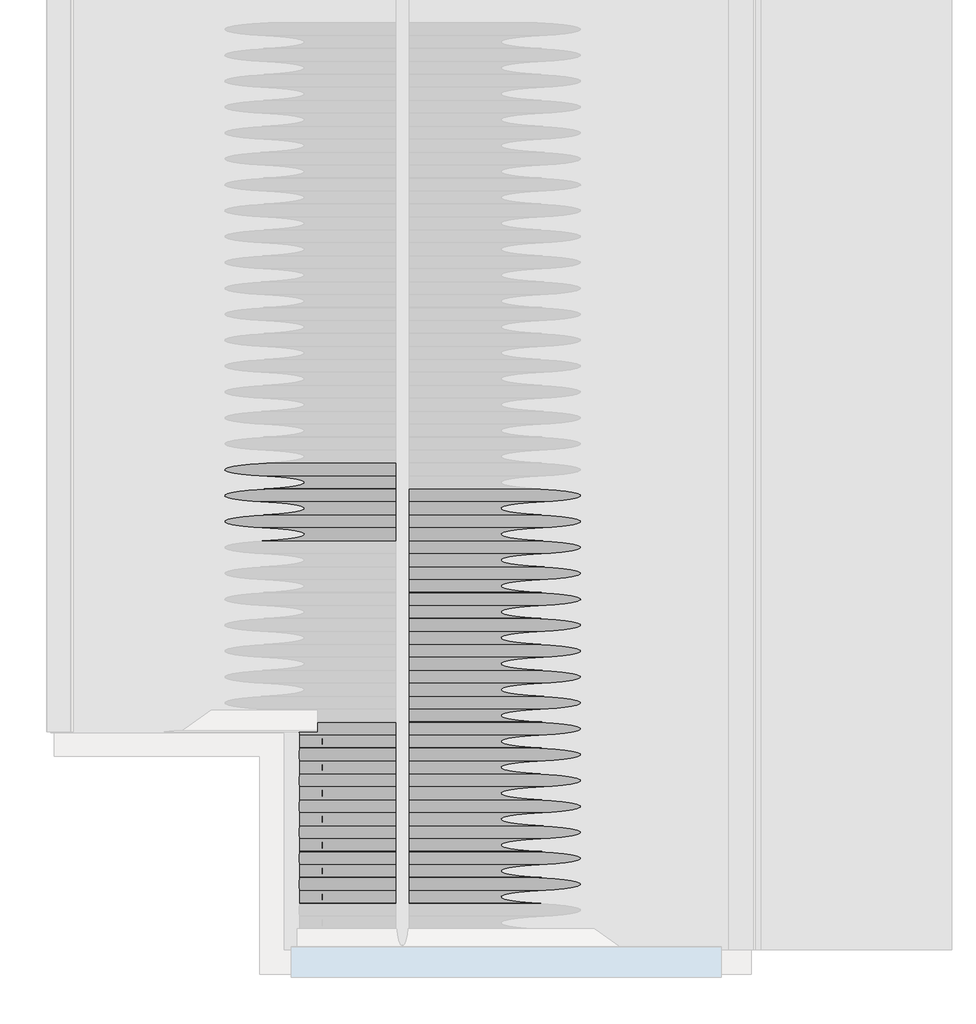
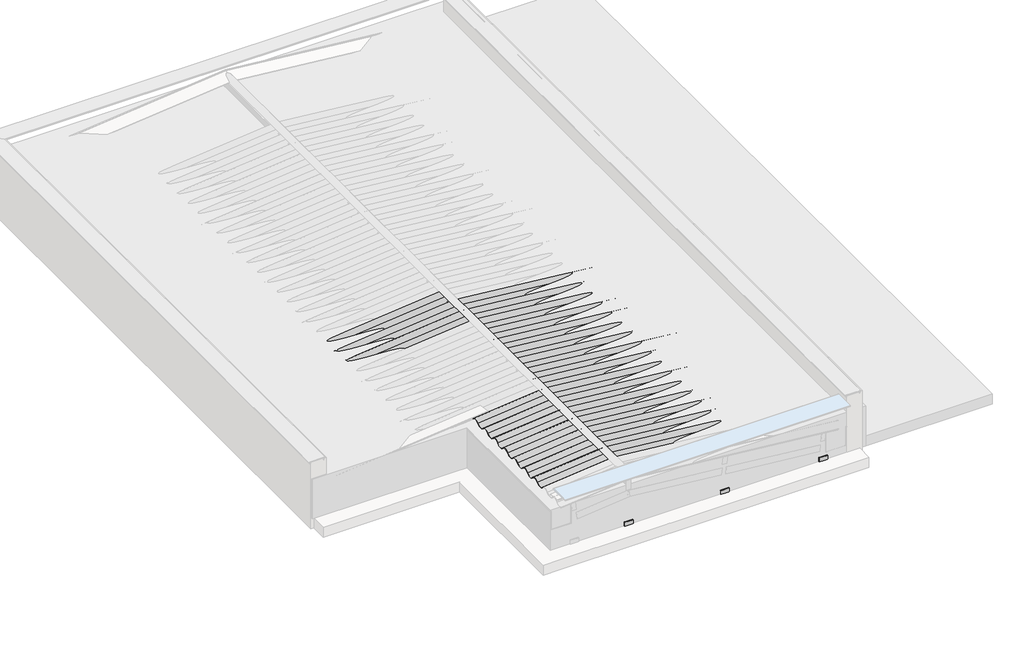
# One storey, part 2 of 4: 34 beams, 4 columns.
"""IFC4 building model written with IfcOpenShell, lengths in millimetres."""

import ifcopenshell
import ifcopenshell.guid

model = None  # the IFC model being written
_history = None  # IfcOwnerHistory: only IFC2X3 demands one
_inside = {}  # id of a spatial element -> (the spatial element, [elements in it])
_under = {}  # id of a project, library or spatial element -> (it, [spatial elements below it])
_declared = {}  # id of a project -> (the project, [libraries it declares])
_typed = {}  # id of a type object -> (the type object, [elements of that type])
_made_of = {}  # id of a material, layer set ... -> (it, [elements and type objects made of it])


def new_model(schema):
    """Start an empty IFC model of exactly this schema.

    Asked for "IFC4X3", IfcOpenShell would pick the latest addendum, in which some entities
    have other attributes; the version numbers below select the first issue.
    IFC2X3 requires an IfcOwnerHistory on every rooted entity: one is made here for all.
    """
    global model, _history
    if schema == "IFC4X3":
        model = ifcopenshell.file(schema_version=(4, 3, 0, 0))
    else:
        model = ifcopenshell.file(schema=schema)
    _inside.clear()
    _under.clear()
    _declared.clear()
    _typed.clear()
    _made_of.clear()
    _history = None
    if model.schema == "IFC2X3":
        org = make("IfcOrganization", Name="unknown")
        user = make(
            "IfcPersonAndOrganization",
            ThePerson=make("IfcPerson", FamilyName="unknown"),
            TheOrganization=org,
        )
        app = make(
            "IfcApplication",
            ApplicationDeveloper=org,
            Version="unknown",
            ApplicationFullName="unknown",
            ApplicationIdentifier="unknown",
        )
        _history = make(
            "IfcOwnerHistory",
            OwningUser=user,
            OwningApplication=app,
            ChangeAction="ADDED",
            CreationDate=0,
        )
    return model


def make(cls, **values):
    """One entity of the class cls with the attributes given. An attribute that is None is left unset."""
    return model.create_entity(
        cls, **{name: value for name, value in values.items() if value is not None}
    )


def rooted(cls, **values):
    """An entity with a GlobalId (a new one), such as an element, a storey or a relation."""
    return make(cls, GlobalId=ifcopenshell.guid.new(), OwnerHistory=_history, **values)


def si_unit(unit_type, name, prefix=None):
    """IfcSIUnit, for example si_unit("LENGTHUNIT", "METRE", prefix="MILLI")."""
    return make("IfcSIUnit", UnitType=unit_type, Prefix=prefix, Name=name)


def assignment(units):
    """IfcUnitAssignment: the units of a project."""
    return None if units is None else make("IfcUnitAssignment", Units=units)


def point(xyz):
    """IfcCartesianPoint."""
    return None if xyz is None else make("IfcCartesianPoint", Coordinates=xyz)


def direction(xyz):
    """IfcDirection."""
    return None if xyz is None else make("IfcDirection", DirectionRatios=xyz)


def frame(location, z_axis=None, x_axis=None):
    """IfcAxis2Placement3D, a coordinate frame: its origin and axes. An axis left out is left unset."""
    return make(
        "IfcAxis2Placement3D",
        Location=point(location),
        Axis=direction(z_axis),
        RefDirection=direction(x_axis),
    )


def frame_2d(location, x_axis=None):
    """IfcAxis2Placement2D, a coordinate frame in the plane: its origin and x axis."""
    return make(
        "IfcAxis2Placement2D", Location=point(location), RefDirection=direction(x_axis)
    )


def origin():
    """The frame at (0, 0, 0) with its axes left unset."""
    return frame((0.0, 0.0, 0.0))


def place(relative_to, where):
    """IfcLocalPlacement: puts the frame where relative to a parent placement (None: the world)."""
    return make(
        "IfcLocalPlacement", PlacementRelTo=relative_to, RelativePlacement=where
    )


def context(
    kind, dimensions, precision=None, world=None, true_north=None, identifier=None
):
    """IfcGeometricRepresentationContext, for example the 3D "Model" context."""
    return make(
        "IfcGeometricRepresentationContext",
        ContextIdentifier=identifier,
        ContextType=kind,
        CoordinateSpaceDimension=dimensions,
        Precision=precision,
        WorldCoordinateSystem=world,
        TrueNorth=true_north,
    )


def project(units=None, contexts=None):
    """IfcProject with its units and contexts."""
    return rooted(
        "IfcProject",
        Name="project",
        RepresentationContexts=contexts,
        UnitsInContext=assignment(units),
    )


def spatial(cls, under=None, at=None, **own):
    """A site, building, storey or space (cls), placed at a placement, below another one or the project."""
    s = rooted(cls, ObjectPlacement=at, **own)
    if under is not None:
        _under.setdefault(under.id(), (under, []))[1].append(s)
    return s


def polyline(points):
    """IfcPolyline through the points."""
    return make("IfcPolyline", Points=[point(p) for p in points])


def circle_curve(where, radius):
    """IfcCircle in the frame where."""
    return make("IfcCircle", Position=where, Radius=radius)


def trimmed(basis, trim1, trim2, sense, master):
    """IfcTrimmedCurve: the piece of a basis curve between two trims."""
    return make(
        "IfcTrimmedCurve",
        BasisCurve=basis,
        Trim1=trim1,
        Trim2=trim2,
        SenseAgreement=sense,
        MasterRepresentation=master,
    )


def segment(curve, same_sense, transition):
    """IfcCompositeCurveSegment."""
    return make(
        "IfcCompositeCurveSegment",
        Transition=transition,
        SameSense=same_sense,
        ParentCurve=curve,
    )


def composite_curve(segments, self_intersect=None):
    """IfcCompositeCurve: segments joined end to end."""
    return make("IfcCompositeCurve", Segments=segments, SelfIntersect=self_intersect)


def outline(outer, holes=None, kind="AREA"):
    """IfcArbitraryClosedProfileDef: a profile drawn as a closed curve; with holes, ...WithVoids."""
    if holes is None:
        return make("IfcArbitraryClosedProfileDef", ProfileType=kind, OuterCurve=outer)
    return make(
        "IfcArbitraryProfileDefWithVoids",
        ProfileType=kind,
        OuterCurve=outer,
        InnerCurves=holes,
    )


def extrude(swept, where, along, depth):
    """IfcExtrudedAreaSolid: the profile swept, set in the frame where, extruded along a direction by depth."""
    return make(
        "IfcExtrudedAreaSolid",
        SweptArea=swept,
        Position=where,
        ExtrudedDirection=direction(along),
        Depth=depth,
    )


def shape(context_of_items, identifier, shape_type, items):
    """IfcShapeRepresentation: the items that make up one representation, for example the "Body"."""
    return make(
        "IfcShapeRepresentation",
        ContextOfItems=context_of_items,
        RepresentationIdentifier=identifier,
        RepresentationType=shape_type,
        Items=items,
    )


def source(mapping_origin, context_of_items, identifier, shape_type, items):
    """IfcRepresentationMap: a shape defined once, which mapped items show again and again."""
    return make(
        "IfcRepresentationMap",
        MappingOrigin=mapping_origin,
        MappedRepresentation=shape(context_of_items, identifier, shape_type, items),
    )


def transform(
    local_origin,
    x_axis=None,
    y_axis=None,
    z_axis=None,
    scale=None,
    scale2=None,
    scale3=None,
    uniform=True,
):
    """IfcCartesianTransformationOperator3D, or its non-uniform kind. x_axis, y_axis, z_axis: its Axis1, 2, 3."""
    if uniform:
        return make(
            "IfcCartesianTransformationOperator3D",
            Axis1=direction(x_axis),
            Axis2=direction(y_axis),
            LocalOrigin=point(local_origin),
            Scale=scale,
            Axis3=direction(z_axis),
        )
    return make(
        "IfcCartesianTransformationOperator3DnonUniform",
        Axis1=direction(x_axis),
        Axis2=direction(y_axis),
        LocalOrigin=point(local_origin),
        Scale=scale,
        Axis3=direction(z_axis),
        Scale2=scale2,
        Scale3=scale3,
    )


def mapped(mapping_source, mapping_target):
    """IfcMappedItem: shows the shape of a source again, moved by a transform."""
    return make(
        "IfcMappedItem", MappingSource=mapping_source, MappingTarget=mapping_target
    )


def made_of(thing, what):
    """Note that an element or type object is made of a material, layer set ...; save() writes the relation."""
    if what is not None:
        _made_of.setdefault(what.id(), (what, []))[1].append(thing)
    return thing


def element(
    cls,
    number,
    at=None,
    inside=None,
    cuts=None,
    type_object=None,
    material=None,
    context=None,
    identifier="Body",
    shape_type=None,
    held_by="IfcProductDefinitionShape",
    body=None,
    shapes=None,
    **own,
):
    """One element of the class cls, such as IfcWall. Its Tag is "e" and its number.

    at: its placement. inside: the storey or other place that contains it. cuts: it is an
    opening in that element (IfcRelVoidsElement). A single representation is given by context,
    identifier, shape_type and body (its items); several are given by shapes. held_by: the class
    of the entity that holds the representations. save() writes the other relations.
    """
    e = rooted(cls, Tag="e%d" % number, ObjectPlacement=at, **own)
    if body is not None:
        shapes = [shape(context, identifier, shape_type, body)]
    if shapes is not None:
        e.Representation = make(held_by, Representations=shapes)
    if inside is not None:
        _inside.setdefault(inside.id(), (inside, []))[1].append(e)
    if cuts is not None:
        rooted(
            "IfcRelVoidsElement", RelatingBuildingElement=cuts, RelatedOpeningElement=e
        )
    if type_object is not None:
        _typed.setdefault(type_object.id(), (type_object, []))[1].append(e)
    return made_of(e, material)


def aggregate(whole, parts):
    """IfcRelAggregates: a whole, such as a stair, and the parts it consists of."""
    return rooted("IfcRelAggregates", RelatingObject=whole, RelatedObjects=parts)


def save(model, path):
    """Write the relations noted so far, then the file.

    IfcRelAggregates (storeys below a building ...), IfcRelContainedInSpatialStructure (elements
    in a storey), IfcRelDefinesByType, IfcRelAssociatesMaterial and IfcRelDeclares: one each for
    every whole, place, type object, material and project.
    """
    for whole, parts in _under.values():
        aggregate(whole, parts)
    for where, things in _inside.values():
        rooted(
            "IfcRelContainedInSpatialStructure",
            RelatedElements=things,
            RelatingStructure=where,
        )
    for kind, things in _typed.values():
        rooted("IfcRelDefinesByType", RelatedObjects=things, RelatingType=kind)
    for what, things in _made_of.values():
        rooted("IfcRelAssociatesMaterial", RelatedObjects=things, RelatingMaterial=what)
    for by, libraries in _declared.values():
        rooted("IfcRelDeclares", RelatingContext=by, RelatedDefinitions=libraries)
    model.write(path)


def column_7d6827b5(model_context):
    return source(origin(), model_context, "Body", "SweptSolid", [
        extrude(outline(polyline([(30.0, 80.0), (30.0, -80.0), (-30.0, -80.0), (-30.0, 80.0), (30.0, 80.0)])), frame((0.0, 0.0, 4460.0), z_axis=(0.0, 0.0, 1.0), x_axis=(1.0, 0.0, 0.0)), (0.0, 0.0, 1.0), 466.0),
    ])


def column_c7348c99(model_context):
    return source(origin(), model_context, "Body", "SweptSolid", [
        extrude(outline(polyline([(30.0, 80.0), (30.0, -80.0), (-30.0, -80.0), (-30.0, 80.0), (30.0, 80.0)])), frame((0.0, 0.0, 4460.0), z_axis=(0.0, 0.0, 1.0), x_axis=(1.0, 0.0, 0.0)), (0.0, 0.0, 1.0), 372.8),
    ])


def column_6cc9e01b(model_context):
    return source(origin(), model_context, "Body", "SweptSolid", [
        extrude(outline(polyline([(30.0, 80.0), (30.0, -80.0), (-30.0, -80.0), (-30.0, 80.0), (30.0, 80.0)])), frame((0.0, 0.0, 4460.0), z_axis=(0.0, 0.0, 1.0), x_axis=(1.0, 0.0, 0.0)), (0.0, 0.0, 1.0), 233.0),
    ])


model = new_model("IFC4")

# Units and contexts
model_context = context("Model", 3, world=origin())
ifc_project = project(units=[si_unit("LENGTHUNIT", "METRE", prefix="MILLI")], contexts=[model_context])

# Site, building, storey
site = spatial("IfcSite", under=ifc_project)
building = spatial("IfcBuilding", under=site)
storey = spatial("IfcBuildingStorey", under=building, Name="COB. SALA ESTAR", Elevation=4400.0)

# Beams
placement = place(None, origin())
element("IfcBeam", 1, ObjectType="Madeira de lei : Berço 6x12cm", at=placement, inside=storey, context=model_context, shape_type="SweptSolid", body=[
    extrude(outline(polyline([(-3400.8557491, 180.4300153), (-3280.8557491, 180.4300153), (-3280.8557491, -1819.5699847), (-3400.8557491, -1819.5699847), (-3400.8557491, 180.4300153)])), frame((0.0, 0.0, 4400.0), z_axis=(0.0, 0.0, 1.0), x_axis=(1.0, 0.0, 0.0)), (0.0, 0.0, 1.0), 60.0),
])
element("IfcBeam", 2, ObjectType="Madeira de lei : Berço 6x12cm", at=placement, inside=storey, context=model_context, shape_type="SweptSolid", body=[
    extrude(outline(polyline([(-3400.8557491, -1819.5699847), (-3280.8557491, -1819.5699847), (-3280.8557491, -4359.5699847), (-3400.8557491, -4359.5699847), (-3400.8557491, -1819.5699847)])), frame((0.0, 0.0, 4400.0), z_axis=(0.0, 0.0, 1.0), x_axis=(1.0, 0.0, 0.0)), (0.0, 0.0, 1.0), 60.0),
])
element("IfcBeam", 3, ObjectType="Madeira de lei : Berço 6x12cm", at=placement, inside=storey, context=model_context, shape_type="SweptSolid", body=[
    extrude(outline(polyline([(-2032.3324227, 180.4300153), (-1912.3324227, 180.4300153), (-1912.3324227, -1819.5699847), (-2032.3324227, -1819.5699847), (-2032.3324227, 180.4300153)])), frame((0.0, 0.0, 4400.0), z_axis=(0.0, 0.0, 1.0), x_axis=(1.0, 0.0, 0.0)), (0.0, 0.0, 1.0), 60.0),
])
element("IfcBeam", 4, ObjectType="Madeira de lei : Berço 6x12cm", at=placement, inside=storey, context=model_context, shape_type="SweptSolid", body=[
    extrude(outline(polyline([(-2032.3324227, -1819.5699847), (-1912.3324227, -1819.5699847), (-1912.3324227, -4359.5699847), (-2032.3324227, -4359.5699847), (-2032.3324227, -1819.5699847)])), frame((0.0, 0.0, 4400.0), z_axis=(0.0, 0.0, 1.0), x_axis=(1.0, 0.0, 0.0)), (0.0, 0.0, 1.0), 60.0),
])
element("IfcBeam", 5, ObjectType="Madeira de lei : Berço 6x12cm", at=placement, inside=storey, context=model_context, shape_type="SweptSolid", body=[
    extrude(outline(polyline([(-634.0324227, 180.4300153), (-514.0324227, 180.4300153), (-514.0324227, -1819.5699847), (-634.0324227, -1819.5699847), (-634.0324227, 180.4300153)])), frame((0.0, 0.0, 4400.0), z_axis=(0.0, 0.0, 1.0), x_axis=(1.0, 0.0, 0.0)), (0.0, 0.0, 1.0), 60.0),
])
element("IfcBeam", 6, ObjectType="Madeira de lei : Berço 6x12cm", at=placement, inside=storey, context=model_context, shape_type="SweptSolid", body=[
    extrude(outline(polyline([(-634.0324227, -1819.5699847), (-514.0324227, -1819.5699847), (-514.0324227, -4359.5699847), (-634.0324227, -4359.5699847), (-634.0324227, -1819.5699847)])), frame((0.0, 0.0, 4400.0), z_axis=(0.0, 0.0, 1.0), x_axis=(1.0, 0.0, 0.0)), (0.0, 0.0, 1.0), 60.0),
])
element("IfcBeam", 7, ObjectType="Madeira de lei : Berço 6x12cm", at=placement, inside=storey, context=model_context, shape_type="SweptSolid", body=[
    extrude(outline(polyline([(-6167.5301913, 2180.4300147), (-6047.5301913, 2180.4300147), (-6047.5301913, 180.4300153), (-6167.5301913, 180.4300153), (-6167.5301913, 2180.4300147)])), frame((0.0, 0.0, 4400.0), z_axis=(0.0, 0.0, 1.0), x_axis=(1.0, 0.0, 0.0)), (0.0, 0.0, 1.0), 60.0),
])
element("IfcBeam", 8, ObjectType="Madeira de lei : Berço 6x12cm", at=placement, inside=storey, context=model_context, shape_type="SweptSolid", body=[
    extrude(outline(polyline([(-4769.2301913, 180.4300153), (-4649.2301913, 180.4300153), (-4649.2301913, -1819.5699847), (-4769.2301913, -1819.5699847), (-4769.2301913, 180.4300153)])), frame((0.0, 0.0, 4400.0), z_axis=(0.0, 0.0, 1.0), x_axis=(1.0, 0.0, 0.0)), (0.0, 0.0, 1.0), 60.0),
])
element("IfcBeam", 9, ObjectType="Telha Ondulada : Fibrocimento", at=placement, inside=storey, context=model_context, shape_type="SweptSolid", body=[
    extrude(outline(composite_curve([segment(trimmed(circle_curve(frame_2d((-58.7002979, -53.2060538)), 66.7939461), [point((-29.3501489, 6.7939462))], [point((-29.3501489, -113.2060538))], False, "CARTESIAN"), True, "CONTINUOUS"), segment(polyline([(-29.3501489, -113.2060538), (-31.5472155, -108.7146288)]), True, "CONTINUOUS"), segment(trimmed(circle_curve(frame_2d((-58.7002979, -53.2060538)), 61.7939461), [point((-31.5472155, -108.7146288))], [point((-31.5472155, 2.3025211))], True, "CARTESIAN"), True, "CONTINUOUS"), segment(trimmed(circle_curve(frame_2d((0.0, 66.7939462)), 71.7939461), [point((-31.5472155, 2.3025211))], [point((-31.5472155, 131.2853712))], False, "CARTESIAN"), True, "CONTINUOUS"), segment(polyline([(-31.5472155, 131.2853712), (-29.3501489, 126.7939462)]), True, "CONTINUOUS"), segment(trimmed(circle_curve(frame_2d((0.0, 66.7939462)), 66.7939461), [point((-29.3501489, 126.7939462))], [point((-29.3501489, 6.7939462))], True, "CARTESIAN"), True, "CONTINUOUS")], self_intersect=False)), frame((-4315.8870688, -3778.673052, 5061.8999542), z_axis=(0.9950371902099892, 0.0, 0.09950371902099964), x_axis=(-0.09950371902099964, 0.0, 0.9950371902099892)), (0.0, 0.0, 1.0), 970.7897678),
])
element("IfcBeam", 10, ObjectType="Telha Ondulada : Fibrocimento", at=placement, inside=storey, context=model_context, shape_type="SweptSolid", body=[
    extrude(outline(composite_curve([segment(trimmed(circle_curve(frame_2d((-58.7002979, -53.2060538)), 66.7939461), [point((-29.3501489, 6.7939462))], [point((-29.3501489, -113.2060538))], False, "CARTESIAN"), True, "CONTINUOUS"), segment(polyline([(-29.3501489, -113.2060538), (-31.5472155, -108.7146288)]), True, "CONTINUOUS"), segment(trimmed(circle_curve(frame_2d((-58.7002979, -53.2060538)), 61.7939461), [point((-31.5472155, -108.7146288))], [point((-31.5472155, 2.3025211))], True, "CARTESIAN"), True, "CONTINUOUS"), segment(trimmed(circle_curve(frame_2d((0.0, 66.7939462)), 71.7939461), [point((-31.5472155, 2.3025211))], [point((-31.5472155, 131.2853712))], False, "CARTESIAN"), True, "CONTINUOUS"), segment(polyline([(-31.5472155, 131.2853712), (-29.3501489, 126.7939462)]), True, "CONTINUOUS"), segment(trimmed(circle_curve(frame_2d((0.0, 66.7939462)), 66.7939461), [point((-29.3501489, 126.7939462))], [point((-29.3501489, 6.7939462))], True, "CARTESIAN"), True, "CONTINUOUS")], self_intersect=False)), frame((-4315.8870688, -3534.173052, 5061.8999542), z_axis=(0.9950371902099892, 0.0, 0.09950371902099958), x_axis=(-0.09950371902099958, 0.0, 0.9950371902099892)), (0.0, 0.0, 1.0), 970.7897678),
])
element("IfcBeam", 11, ObjectType="Telha Ondulada : Fibrocimento", at=placement, inside=storey, context=model_context, shape_type="SweptSolid", body=[
    extrude(outline(composite_curve([segment(trimmed(circle_curve(frame_2d((-58.7002979, -53.2060538)), 66.7939461), [point((-29.3501489, 6.7939462))], [point((-29.3501489, -113.2060538))], False, "CARTESIAN"), True, "CONTINUOUS"), segment(polyline([(-29.3501489, -113.2060538), (-31.5472155, -108.7146288)]), True, "CONTINUOUS"), segment(trimmed(circle_curve(frame_2d((-58.7002979, -53.2060538)), 61.7939461), [point((-31.5472155, -108.7146288))], [point((-31.5472155, 2.3025211))], True, "CARTESIAN"), True, "CONTINUOUS"), segment(trimmed(circle_curve(frame_2d((0.0, 66.7939462)), 71.7939461), [point((-31.5472155, 2.3025211))], [point((-31.5472155, 131.2853712))], False, "CARTESIAN"), True, "CONTINUOUS"), segment(polyline([(-31.5472155, 131.2853712), (-29.3501489, 126.7939462)]), True, "CONTINUOUS"), segment(trimmed(circle_curve(frame_2d((0.0, 66.7939462)), 66.7939461), [point((-29.3501489, 126.7939462))], [point((-29.3501489, 6.7939462))], True, "CARTESIAN"), True, "CONTINUOUS")], self_intersect=False)), frame((-4315.8870688, -3289.673052, 5061.8999542), z_axis=(0.9950371902099892, 0.0, 0.09950371902099958), x_axis=(-0.09950371902099958, 0.0, 0.9950371902099892)), (0.0, 0.0, 1.0), 970.7897678),
])
element("IfcBeam", 12, ObjectType="Telha Ondulada : Fibrocimento", at=placement, inside=storey, context=model_context, shape_type="SweptSolid", body=[
    extrude(outline(composite_curve([segment(trimmed(circle_curve(frame_2d((-58.7002979, -53.2060538)), 66.7939461), [point((-29.3501489, 6.7939462))], [point((-29.3501489, -113.2060538))], False, "CARTESIAN"), True, "CONTINUOUS"), segment(polyline([(-29.3501489, -113.2060538), (-31.5472155, -108.7146288)]), True, "CONTINUOUS"), segment(trimmed(circle_curve(frame_2d((-58.7002979, -53.2060538)), 61.7939461), [point((-31.5472155, -108.7146288))], [point((-31.5472155, 2.3025211))], True, "CARTESIAN"), True, "CONTINUOUS"), segment(trimmed(circle_curve(frame_2d((0.0, 66.7939462)), 71.7939461), [point((-31.5472155, 2.3025211))], [point((-31.5472155, 131.2853712))], False, "CARTESIAN"), True, "CONTINUOUS"), segment(polyline([(-31.5472155, 131.2853712), (-29.3501489, 126.7939462)]), True, "CONTINUOUS"), segment(trimmed(circle_curve(frame_2d((0.0, 66.7939462)), 66.7939461), [point((-29.3501489, 126.7939462))], [point((-29.3501489, 6.7939462))], True, "CARTESIAN"), True, "CONTINUOUS")], self_intersect=False)), frame((-4315.8870688, -3045.173052, 5061.8999542), z_axis=(0.9950371902099892, 0.0, 0.09950371902099958), x_axis=(-0.09950371902099958, 0.0, 0.9950371902099892)), (0.0, 0.0, 1.0), 970.7897678),
])
element("IfcBeam", 13, ObjectType="Telha Ondulada : Fibrocimento", at=placement, inside=storey, context=model_context, shape_type="SweptSolid", body=[
    extrude(outline(composite_curve([segment(trimmed(circle_curve(frame_2d((-58.7002979, -53.2060538)), 66.7939461), [point((-29.3501489, 6.7939462))], [point((-29.3501489, -113.2060538))], False, "CARTESIAN"), True, "CONTINUOUS"), segment(polyline([(-29.3501489, -113.2060538), (-31.5472155, -108.7146288)]), True, "CONTINUOUS"), segment(trimmed(circle_curve(frame_2d((-58.7002979, -53.2060538)), 61.7939461), [point((-31.5472155, -108.7146288))], [point((-31.5472155, 2.3025211))], True, "CARTESIAN"), True, "CONTINUOUS"), segment(trimmed(circle_curve(frame_2d((0.0, 66.7939462)), 71.7939461), [point((-31.5472155, 2.3025211))], [point((-31.5472155, 131.2853712))], False, "CARTESIAN"), True, "CONTINUOUS"), segment(polyline([(-31.5472155, 131.2853712), (-29.3501489, 126.7939462)]), True, "CONTINUOUS"), segment(trimmed(circle_curve(frame_2d((0.0, 66.7939462)), 66.7939461), [point((-29.3501489, 126.7939462))], [point((-29.3501489, 6.7939462))], True, "CARTESIAN"), True, "CONTINUOUS")], self_intersect=False)), frame((-4315.8870688, -2800.673052, 5061.8999542), z_axis=(0.9950371902099892, 0.0, 0.09950371902099964), x_axis=(-0.09950371902099964, 0.0, 0.9950371902099892)), (0.0, 0.0, 1.0), 970.7897678),
])
element("IfcBeam", 14, ObjectType="Telha Ondulada : Fibrocimento", at=placement, inside=storey, context=model_context, shape_type="SweptSolid", body=[
    extrude(outline(composite_curve([segment(trimmed(circle_curve(frame_2d((-58.7002979, -53.2060538)), 66.7939461), [point((-29.3501489, 6.7939462))], [point((-29.3501489, -113.2060538))], False, "CARTESIAN"), True, "CONTINUOUS"), segment(polyline([(-29.3501489, -113.2060538), (-31.5472155, -108.7146288)]), True, "CONTINUOUS"), segment(trimmed(circle_curve(frame_2d((-58.7002979, -53.2060538)), 61.7939461), [point((-31.5472155, -108.7146288))], [point((-31.5472155, 2.3025211))], True, "CARTESIAN"), True, "CONTINUOUS"), segment(trimmed(circle_curve(frame_2d((0.0, 66.7939462)), 71.7939461), [point((-31.5472155, 2.3025211))], [point((-31.5472155, 131.2853712))], False, "CARTESIAN"), True, "CONTINUOUS"), segment(polyline([(-31.5472155, 131.2853712), (-29.3501489, 126.7939462)]), True, "CONTINUOUS"), segment(trimmed(circle_curve(frame_2d((0.0, 66.7939462)), 66.7939461), [point((-29.3501489, 126.7939462))], [point((-29.3501489, 6.7939462))], True, "CARTESIAN"), True, "CONTINUOUS")], self_intersect=False)), frame((-4315.8870688, -2556.173052, 5061.8999542), z_axis=(0.9950371902099892, 0.0, 0.09950371902099969), x_axis=(-0.09950371902099969, 0.0, 0.9950371902099892)), (0.0, 0.0, 1.0), 970.7897678),
])
element("IfcBeam", 15, ObjectType="Telha Ondulada : Fibrocimento", at=placement, inside=storey, context=model_context, shape_type="SweptSolid", body=[
    extrude(outline(composite_curve([segment(trimmed(circle_curve(frame_2d((-58.7002979, -53.2060538)), 66.7939461), [point((-29.3501489, 6.7939462))], [point((-29.3501489, -113.2060538))], False, "CARTESIAN"), True, "CONTINUOUS"), segment(polyline([(-29.3501489, -113.2060538), (-31.5472155, -108.7146288)]), True, "CONTINUOUS"), segment(trimmed(circle_curve(frame_2d((-58.7002979, -53.2060538)), 61.7939461), [point((-31.5472155, -108.7146288))], [point((-31.5472155, 2.3025211))], True, "CARTESIAN"), True, "CONTINUOUS"), segment(trimmed(circle_curve(frame_2d((0.0, 66.7939462)), 71.7939461), [point((-31.5472155, 2.3025211))], [point((-31.5472155, 131.2853712))], False, "CARTESIAN"), True, "CONTINUOUS"), segment(polyline([(-31.5472155, 131.2853712), (-29.3501489, 126.7939462)]), True, "CONTINUOUS"), segment(trimmed(circle_curve(frame_2d((0.0, 66.7939462)), 66.7939461), [point((-29.3501489, 126.7939462))], [point((-29.3501489, 6.7939462))], True, "CARTESIAN"), True, "CONTINUOUS")], self_intersect=False)), frame((-4315.8870688, -2311.673052, 5061.8999542), z_axis=(0.9950371902099892, 0.0, 0.09950371902099958), x_axis=(-0.09950371902099958, 0.0, 0.9950371902099892)), (0.0, 0.0, 1.0), 970.7897678),
])
element("IfcBeam", 16, ObjectType="Telha Ondulada : Fibrocimento", at=placement, inside=storey, context=model_context, shape_type="SweptSolid", body=[
    extrude(outline(composite_curve([segment(trimmed(circle_curve(frame_2d((-58.7002978, -53.2060538)), 66.7939461), [point((-29.3501489, 6.7939462))], [point((-29.3501489, -113.2060538))], False, "CARTESIAN"), True, "CONTINUOUS"), segment(polyline([(-29.3501489, -113.2060538), (-31.5472154, -108.7146288)]), True, "CONTINUOUS"), segment(trimmed(circle_curve(frame_2d((-58.7002978, -53.2060538)), 61.7939461), [point((-31.5472154, -108.7146288))], [point((-31.5472154, 2.3025211))], True, "CARTESIAN"), True, "CONTINUOUS"), segment(trimmed(circle_curve(frame_2d((0.0, 66.7939462)), 71.7939461), [point((-31.5472154, 2.3025211))], [point((-31.5472154, 131.2853712))], False, "CARTESIAN"), True, "CONTINUOUS"), segment(polyline([(-31.5472154, 131.2853712), (-29.3501489, 126.7939462)]), True, "CONTINUOUS"), segment(trimmed(circle_curve(frame_2d((0.0, 66.7939462)), 66.7939461), [point((-29.3501489, 126.7939462))], [point((-29.3501489, 6.7939462))], True, "CARTESIAN"), True, "CONTINUOUS")], self_intersect=False)), frame((-6307.6707245, -355.673052, 4862.7215886), z_axis=(0.9950371902099892, 0.0, 0.09950371902099968), x_axis=(-0.09950371902099968, 0.0, 0.9950371902099892)), (0.0, 0.0, 1.0), 2972.5075682),
])
element("IfcBeam", 17, ObjectType="Telha Ondulada : Fibrocimento", at=placement, inside=storey, context=model_context, shape_type="SweptSolid", body=[
    extrude(outline(composite_curve([segment(trimmed(circle_curve(frame_2d((-58.7002978, -53.2060538)), 66.7939461), [point((-29.3501489, 6.7939462))], [point((-29.3501489, -113.2060538))], False, "CARTESIAN"), True, "CONTINUOUS"), segment(polyline([(-29.3501489, -113.2060538), (-31.5472154, -108.7146288)]), True, "CONTINUOUS"), segment(trimmed(circle_curve(frame_2d((-58.7002978, -53.2060538)), 61.7939461), [point((-31.5472154, -108.7146288))], [point((-31.5472154, 2.3025211))], True, "CARTESIAN"), True, "CONTINUOUS"), segment(trimmed(circle_curve(frame_2d((0.0, 66.7939462)), 71.7939461), [point((-31.5472154, 2.3025211))], [point((-31.5472154, 131.2853712))], False, "CARTESIAN"), True, "CONTINUOUS"), segment(polyline([(-31.5472154, 131.2853712), (-29.3501489, 126.7939462)]), True, "CONTINUOUS"), segment(trimmed(circle_curve(frame_2d((0.0, 66.7939462)), 66.7939461), [point((-29.3501489, 126.7939462))], [point((-29.3501489, 6.7939462))], True, "CARTESIAN"), True, "CONTINUOUS")], self_intersect=False)), frame((-6307.6707245, -111.173052, 4862.7215886), z_axis=(0.9950371902099892, 0.0, 0.09950371902099969), x_axis=(-0.09950371902099969, 0.0, 0.9950371902099892)), (0.0, 0.0, 1.0), 2972.5075682),
])
element("IfcBeam", 18, ObjectType="Telha Ondulada : Fibrocimento", at=placement, inside=storey, context=model_context, shape_type="SweptSolid", body=[
    extrude(outline(composite_curve([segment(trimmed(circle_curve(frame_2d((-58.7002978, -53.2060538)), 66.7939461), [point((-29.3501489, 6.7939462))], [point((-29.3501489, -113.2060538))], False, "CARTESIAN"), True, "CONTINUOUS"), segment(polyline([(-29.3501489, -113.2060538), (-31.5472154, -108.7146288)]), True, "CONTINUOUS"), segment(trimmed(circle_curve(frame_2d((-58.7002978, -53.2060538)), 61.7939461), [point((-31.5472154, -108.7146288))], [point((-31.5472154, 2.3025211))], True, "CARTESIAN"), True, "CONTINUOUS"), segment(trimmed(circle_curve(frame_2d((0.0, 66.7939462)), 71.7939461), [point((-31.5472154, 2.3025211))], [point((-31.5472154, 131.2853712))], False, "CARTESIAN"), True, "CONTINUOUS"), segment(polyline([(-31.5472154, 131.2853712), (-29.3501489, 126.7939462)]), True, "CONTINUOUS"), segment(trimmed(circle_curve(frame_2d((0.0, 66.7939462)), 66.7939461), [point((-29.3501489, 126.7939462))], [point((-29.3501489, 6.7939462))], True, "CARTESIAN"), True, "CONTINUOUS")], self_intersect=False)), frame((-6307.6707245, 133.326948, 4862.7215886), z_axis=(0.9950371902099892, 0.0, 0.09950371902099972), x_axis=(-0.09950371902099972, 0.0, 0.9950371902099892)), (0.0, 0.0, 1.0), 2972.5075682),
])
element("IfcBeam", 19, ObjectType="Telha Ondulada : Fibrocimento", at=placement, inside=storey, context=model_context, shape_type="SweptSolid", body=[
    extrude(outline(composite_curve([segment(trimmed(circle_curve(frame_2d((0.0, 66.7939462)), 66.7939461), [point((29.3501489, 6.7939462))], [point((29.3501489, 126.7939462))], True, "CARTESIAN"), True, "CONTINUOUS"), segment(polyline([(29.3501489, 126.7939462), (31.5472154, 131.2853712)]), True, "CONTINUOUS"), segment(trimmed(circle_curve(frame_2d((0.0, 66.7939462)), 71.7939461), [point((31.5472154, 131.2853712))], [point((31.5472154, 2.3025211))], False, "CARTESIAN"), True, "CONTINUOUS"), segment(trimmed(circle_curve(frame_2d((58.7002978, -53.2060538)), 61.7939461), [point((31.5472154, 2.3025211))], [point((31.5472154, -108.7146288))], True, "CARTESIAN"), True, "CONTINUOUS"), segment(polyline([(31.5472154, -108.7146288), (29.3501489, -113.2060538)]), True, "CONTINUOUS"), segment(trimmed(circle_curve(frame_2d((58.7002978, -53.2060538)), 66.7939461), [point((29.3501489, -113.2060538))], [point((29.3501489, 6.7939462))], False, "CARTESIAN"), True, "CONTINUOUS")], self_intersect=False)), frame((-373.8918894, -3778.673052, 4862.7215886), z_axis=(-0.9950371902099892, 0.0, 0.09950371902099943), x_axis=(-0.09950371902099943, 0.0, -0.9950371902099892)), (0.0, 0.0, 1.0), 2972.5075682),
])
element("IfcBeam", 20, ObjectType="Telha Ondulada : Fibrocimento", at=placement, inside=storey, context=model_context, shape_type="SweptSolid", body=[
    extrude(outline(composite_curve([segment(trimmed(circle_curve(frame_2d((0.0, 66.7939462)), 66.7939461), [point((29.3501489, 6.7939462))], [point((29.3501489, 126.7939462))], True, "CARTESIAN"), True, "CONTINUOUS"), segment(polyline([(29.3501489, 126.7939462), (31.5472154, 131.2853712)]), True, "CONTINUOUS"), segment(trimmed(circle_curve(frame_2d((0.0, 66.7939462)), 71.7939461), [point((31.5472154, 131.2853712))], [point((31.5472154, 2.3025211))], False, "CARTESIAN"), True, "CONTINUOUS"), segment(trimmed(circle_curve(frame_2d((58.7002978, -53.2060538)), 61.7939461), [point((31.5472154, 2.3025211))], [point((31.5472154, -108.7146288))], True, "CARTESIAN"), True, "CONTINUOUS"), segment(polyline([(31.5472154, -108.7146288), (29.3501489, -113.2060538)]), True, "CONTINUOUS"), segment(trimmed(circle_curve(frame_2d((58.7002978, -53.2060538)), 66.7939461), [point((29.3501489, -113.2060538))], [point((29.3501489, 6.7939462))], False, "CARTESIAN"), True, "CONTINUOUS")], self_intersect=False)), frame((-373.8918894, -3534.173052, 4862.7215886), z_axis=(-0.9950371902099892, 0.0, 0.09950371902099943), x_axis=(-0.09950371902099943, 0.0, -0.9950371902099892)), (0.0, 0.0, 1.0), 2972.5075682),
])
element("IfcBeam", 21, ObjectType="Telha Ondulada : Fibrocimento", at=placement, inside=storey, context=model_context, shape_type="SweptSolid", body=[
    extrude(outline(composite_curve([segment(trimmed(circle_curve(frame_2d((0.0, 66.7939462)), 66.7939461), [point((29.3501489, 6.7939462))], [point((29.3501489, 126.7939462))], True, "CARTESIAN"), True, "CONTINUOUS"), segment(polyline([(29.3501489, 126.7939462), (31.5472154, 131.2853712)]), True, "CONTINUOUS"), segment(trimmed(circle_curve(frame_2d((0.0, 66.7939462)), 71.7939461), [point((31.5472154, 131.2853712))], [point((31.5472154, 2.3025211))], False, "CARTESIAN"), True, "CONTINUOUS"), segment(trimmed(circle_curve(frame_2d((58.7002978, -53.2060538)), 61.7939461), [point((31.5472154, 2.3025211))], [point((31.5472154, -108.7146288))], True, "CARTESIAN"), True, "CONTINUOUS"), segment(polyline([(31.5472154, -108.7146288), (29.3501489, -113.2060538)]), True, "CONTINUOUS"), segment(trimmed(circle_curve(frame_2d((58.7002978, -53.2060538)), 66.7939461), [point((29.3501489, -113.2060538))], [point((29.3501489, 6.7939462))], False, "CARTESIAN"), True, "CONTINUOUS")], self_intersect=False)), frame((-373.8918894, -3289.673052, 4862.7215886), z_axis=(-0.9950371902099892, 0.0, 0.09950371902099943), x_axis=(-0.09950371902099943, 0.0, -0.9950371902099892)), (0.0, 0.0, 1.0), 2972.5075682),
])
element("IfcBeam", 22, ObjectType="Telha Ondulada : Fibrocimento", at=placement, inside=storey, context=model_context, shape_type="SweptSolid", body=[
    extrude(outline(composite_curve([segment(trimmed(circle_curve(frame_2d((0.0, 66.7939462)), 66.7939461), [point((29.3501489, 6.7939462))], [point((29.3501489, 126.7939462))], True, "CARTESIAN"), True, "CONTINUOUS"), segment(polyline([(29.3501489, 126.7939462), (31.5472154, 131.2853712)]), True, "CONTINUOUS"), segment(trimmed(circle_curve(frame_2d((0.0, 66.7939462)), 71.7939461), [point((31.5472154, 131.2853712))], [point((31.5472154, 2.3025211))], False, "CARTESIAN"), True, "CONTINUOUS"), segment(trimmed(circle_curve(frame_2d((58.7002978, -53.2060538)), 61.7939461), [point((31.5472154, 2.3025211))], [point((31.5472154, -108.7146288))], True, "CARTESIAN"), True, "CONTINUOUS"), segment(polyline([(31.5472154, -108.7146288), (29.3501489, -113.2060538)]), True, "CONTINUOUS"), segment(trimmed(circle_curve(frame_2d((58.7002978, -53.2060538)), 66.7939461), [point((29.3501489, -113.2060538))], [point((29.3501489, 6.7939462))], False, "CARTESIAN"), True, "CONTINUOUS")], self_intersect=False)), frame((-373.8918894, -3045.173052, 4862.7215886), z_axis=(-0.9950371902099892, 0.0, 0.09950371902099943), x_axis=(-0.09950371902099943, 0.0, -0.9950371902099892)), (0.0, 0.0, 1.0), 2972.5075682),
])
element("IfcBeam", 23, ObjectType="Telha Ondulada : Fibrocimento", at=placement, inside=storey, context=model_context, shape_type="SweptSolid", body=[
    extrude(outline(composite_curve([segment(trimmed(circle_curve(frame_2d((0.0, 66.7939462)), 66.7939461), [point((29.3501489, 6.7939462))], [point((29.3501489, 126.7939462))], True, "CARTESIAN"), True, "CONTINUOUS"), segment(polyline([(29.3501489, 126.7939462), (31.5472154, 131.2853712)]), True, "CONTINUOUS"), segment(trimmed(circle_curve(frame_2d((0.0, 66.7939462)), 71.7939461), [point((31.5472154, 131.2853712))], [point((31.5472154, 2.3025211))], False, "CARTESIAN"), True, "CONTINUOUS"), segment(trimmed(circle_curve(frame_2d((58.7002978, -53.2060538)), 61.7939461), [point((31.5472154, 2.3025211))], [point((31.5472154, -108.7146288))], True, "CARTESIAN"), True, "CONTINUOUS"), segment(polyline([(31.5472154, -108.7146288), (29.3501489, -113.2060538)]), True, "CONTINUOUS"), segment(trimmed(circle_curve(frame_2d((58.7002978, -53.2060538)), 66.7939461), [point((29.3501489, -113.2060538))], [point((29.3501489, 6.7939462))], False, "CARTESIAN"), True, "CONTINUOUS")], self_intersect=False)), frame((-373.8918894, -2800.673052, 4862.7215886), z_axis=(-0.9950371902099892, 0.0, 0.09950371902099943), x_axis=(-0.09950371902099943, 0.0, -0.9950371902099892)), (0.0, 0.0, 1.0), 2972.5075682),
])
element("IfcBeam", 24, ObjectType="Telha Ondulada : Fibrocimento", at=placement, inside=storey, context=model_context, shape_type="SweptSolid", body=[
    extrude(outline(composite_curve([segment(trimmed(circle_curve(frame_2d((0.0, 66.7939462)), 66.7939461), [point((29.3501489, 6.7939462))], [point((29.3501489, 126.7939462))], True, "CARTESIAN"), True, "CONTINUOUS"), segment(polyline([(29.3501489, 126.7939462), (31.5472154, 131.2853712)]), True, "CONTINUOUS"), segment(trimmed(circle_curve(frame_2d((0.0, 66.7939462)), 71.7939461), [point((31.5472154, 131.2853712))], [point((31.5472154, 2.3025211))], False, "CARTESIAN"), True, "CONTINUOUS"), segment(trimmed(circle_curve(frame_2d((58.7002978, -53.2060538)), 61.7939461), [point((31.5472154, 2.3025211))], [point((31.5472154, -108.7146288))], True, "CARTESIAN"), True, "CONTINUOUS"), segment(polyline([(31.5472154, -108.7146288), (29.3501489, -113.2060538)]), True, "CONTINUOUS"), segment(trimmed(circle_curve(frame_2d((58.7002978, -53.2060538)), 66.7939461), [point((29.3501489, -113.2060538))], [point((29.3501489, 6.7939462))], False, "CARTESIAN"), True, "CONTINUOUS")], self_intersect=False)), frame((-373.8918894, -2556.173052, 4862.7215886), z_axis=(-0.9950371902099892, 0.0, 0.09950371902099943), x_axis=(-0.09950371902099943, 0.0, -0.9950371902099892)), (0.0, 0.0, 1.0), 2972.5075682),
])
element("IfcBeam", 25, ObjectType="Telha Ondulada : Fibrocimento", at=placement, inside=storey, context=model_context, shape_type="SweptSolid", body=[
    extrude(outline(composite_curve([segment(trimmed(circle_curve(frame_2d((0.0, 66.7939462)), 66.7939461), [point((29.3501489, 6.7939462))], [point((29.3501489, 126.7939462))], True, "CARTESIAN"), True, "CONTINUOUS"), segment(polyline([(29.3501489, 126.7939462), (31.5472154, 131.2853712)]), True, "CONTINUOUS"), segment(trimmed(circle_curve(frame_2d((0.0, 66.7939462)), 71.7939461), [point((31.5472154, 131.2853712))], [point((31.5472154, 2.3025211))], False, "CARTESIAN"), True, "CONTINUOUS"), segment(trimmed(circle_curve(frame_2d((58.7002978, -53.2060538)), 61.7939461), [point((31.5472154, 2.3025211))], [point((31.5472154, -108.7146288))], True, "CARTESIAN"), True, "CONTINUOUS"), segment(polyline([(31.5472154, -108.7146288), (29.3501489, -113.2060538)]), True, "CONTINUOUS"), segment(trimmed(circle_curve(frame_2d((58.7002978, -53.2060538)), 66.7939461), [point((29.3501489, -113.2060538))], [point((29.3501489, 6.7939462))], False, "CARTESIAN"), True, "CONTINUOUS")], self_intersect=False)), frame((-373.8918894, -2311.673052, 4862.7215886), z_axis=(-0.9950371902099892, 0.0, 0.09950371902099943), x_axis=(-0.09950371902099943, 0.0, -0.9950371902099892)), (0.0, 0.0, 1.0), 2972.5075682),
])
element("IfcBeam", 26, ObjectType="Telha Ondulada : Fibrocimento", at=placement, inside=storey, context=model_context, shape_type="SweptSolid", body=[
    extrude(outline(composite_curve([segment(trimmed(circle_curve(frame_2d((0.0, 66.7939462)), 66.7939461), [point((29.3501489, 6.7939462))], [point((29.3501489, 126.7939462))], True, "CARTESIAN"), True, "CONTINUOUS"), segment(polyline([(29.3501489, 126.7939462), (31.5472154, 131.2853712)]), True, "CONTINUOUS"), segment(trimmed(circle_curve(frame_2d((0.0, 66.7939462)), 71.7939461), [point((31.5472154, 131.2853712))], [point((31.5472154, 2.3025211))], False, "CARTESIAN"), True, "CONTINUOUS"), segment(trimmed(circle_curve(frame_2d((58.7002978, -53.2060538)), 61.7939461), [point((31.5472154, 2.3025211))], [point((31.5472154, -108.7146288))], True, "CARTESIAN"), True, "CONTINUOUS"), segment(polyline([(31.5472154, -108.7146288), (29.3501489, -113.2060538)]), True, "CONTINUOUS"), segment(trimmed(circle_curve(frame_2d((58.7002978, -53.2060538)), 66.7939461), [point((29.3501489, -113.2060538))], [point((29.3501489, 6.7939462))], False, "CARTESIAN"), True, "CONTINUOUS")], self_intersect=False)), frame((-373.8918894, -2067.173052, 4862.7215886), z_axis=(-0.9950371902099892, 0.0, 0.09950371902099943), x_axis=(-0.09950371902099943, 0.0, -0.9950371902099892)), (0.0, 0.0, 1.0), 2972.5075682),
])
element("IfcBeam", 27, ObjectType="Telha Ondulada : Fibrocimento", at=placement, inside=storey, context=model_context, shape_type="SweptSolid", body=[
    extrude(outline(composite_curve([segment(trimmed(circle_curve(frame_2d((0.0, 66.7939462)), 66.7939461), [point((29.3501489, 6.7939462))], [point((29.3501489, 126.7939462))], True, "CARTESIAN"), True, "CONTINUOUS"), segment(polyline([(29.3501489, 126.7939462), (31.5472154, 131.2853712)]), True, "CONTINUOUS"), segment(trimmed(circle_curve(frame_2d((0.0, 66.7939462)), 71.7939461), [point((31.5472154, 131.2853712))], [point((31.5472154, 2.3025211))], False, "CARTESIAN"), True, "CONTINUOUS"), segment(trimmed(circle_curve(frame_2d((58.7002978, -53.2060538)), 61.7939461), [point((31.5472154, 2.3025211))], [point((31.5472154, -108.7146288))], True, "CARTESIAN"), True, "CONTINUOUS"), segment(polyline([(31.5472154, -108.7146288), (29.3501489, -113.2060538)]), True, "CONTINUOUS"), segment(trimmed(circle_curve(frame_2d((58.7002978, -53.2060538)), 66.7939461), [point((29.3501489, -113.2060538))], [point((29.3501489, 6.7939462))], False, "CARTESIAN"), True, "CONTINUOUS")], self_intersect=False)), frame((-373.8918894, -1822.673052, 4862.7215886), z_axis=(-0.9950371902099892, 0.0, 0.09950371902099946), x_axis=(-0.09950371902099946, 0.0, -0.9950371902099892)), (0.0, 0.0, 1.0), 2972.5075682),
])
element("IfcBeam", 28, ObjectType="Telha Ondulada : Fibrocimento", at=placement, inside=storey, context=model_context, shape_type="SweptSolid", body=[
    extrude(outline(composite_curve([segment(trimmed(circle_curve(frame_2d((0.0, 66.7939462)), 66.7939461), [point((29.3501489, 6.7939462))], [point((29.3501489, 126.7939462))], True, "CARTESIAN"), True, "CONTINUOUS"), segment(polyline([(29.3501489, 126.7939462), (31.5472154, 131.2853712)]), True, "CONTINUOUS"), segment(trimmed(circle_curve(frame_2d((0.0, 66.7939462)), 71.7939461), [point((31.5472154, 131.2853712))], [point((31.5472154, 2.3025211))], False, "CARTESIAN"), True, "CONTINUOUS"), segment(trimmed(circle_curve(frame_2d((58.7002978, -53.2060538)), 61.7939461), [point((31.5472154, 2.3025211))], [point((31.5472154, -108.7146288))], True, "CARTESIAN"), True, "CONTINUOUS"), segment(polyline([(31.5472154, -108.7146288), (29.3501489, -113.2060538)]), True, "CONTINUOUS"), segment(trimmed(circle_curve(frame_2d((58.7002978, -53.2060538)), 66.7939461), [point((29.3501489, -113.2060538))], [point((29.3501489, 6.7939462))], False, "CARTESIAN"), True, "CONTINUOUS")], self_intersect=False)), frame((-373.8918894, -1578.173052, 4862.7215886), z_axis=(-0.9950371902099892, 0.0, 0.09950371902099946), x_axis=(-0.09950371902099946, 0.0, -0.9950371902099892)), (0.0, 0.0, 1.0), 2972.5075682),
])
element("IfcBeam", 29, ObjectType="Telha Ondulada : Fibrocimento", at=placement, inside=storey, context=model_context, shape_type="SweptSolid", body=[
    extrude(outline(composite_curve([segment(trimmed(circle_curve(frame_2d((0.0, 66.7939462)), 66.7939461), [point((29.3501489, 6.7939462))], [point((29.3501489, 126.7939462))], True, "CARTESIAN"), True, "CONTINUOUS"), segment(polyline([(29.3501489, 126.7939462), (31.5472154, 131.2853712)]), True, "CONTINUOUS"), segment(trimmed(circle_curve(frame_2d((0.0, 66.7939462)), 71.7939461), [point((31.5472154, 131.2853712))], [point((31.5472154, 2.3025211))], False, "CARTESIAN"), True, "CONTINUOUS"), segment(trimmed(circle_curve(frame_2d((58.7002978, -53.2060538)), 61.7939461), [point((31.5472154, 2.3025211))], [point((31.5472154, -108.7146288))], True, "CARTESIAN"), True, "CONTINUOUS"), segment(polyline([(31.5472154, -108.7146288), (29.3501489, -113.2060538)]), True, "CONTINUOUS"), segment(trimmed(circle_curve(frame_2d((58.7002978, -53.2060538)), 66.7939461), [point((29.3501489, -113.2060538))], [point((29.3501489, 6.7939462))], False, "CARTESIAN"), True, "CONTINUOUS")], self_intersect=False)), frame((-373.8918894, -1333.673052, 4862.7215886), z_axis=(-0.9950371902099892, 0.0, 0.09950371902099946), x_axis=(-0.09950371902099946, 0.0, -0.9950371902099892)), (0.0, 0.0, 1.0), 2972.5075682),
])
element("IfcBeam", 30, ObjectType="Telha Ondulada : Fibrocimento", at=placement, inside=storey, context=model_context, shape_type="SweptSolid", body=[
    extrude(outline(composite_curve([segment(trimmed(circle_curve(frame_2d((0.0, 66.7939462)), 66.7939461), [point((29.3501489, 6.7939462))], [point((29.3501489, 126.7939462))], True, "CARTESIAN"), True, "CONTINUOUS"), segment(polyline([(29.3501489, 126.7939462), (31.5472154, 131.2853712)]), True, "CONTINUOUS"), segment(trimmed(circle_curve(frame_2d((0.0, 66.7939462)), 71.7939461), [point((31.5472154, 131.2853712))], [point((31.5472154, 2.3025211))], False, "CARTESIAN"), True, "CONTINUOUS"), segment(trimmed(circle_curve(frame_2d((58.7002978, -53.2060538)), 61.7939461), [point((31.5472154, 2.3025211))], [point((31.5472154, -108.7146288))], True, "CARTESIAN"), True, "CONTINUOUS"), segment(polyline([(31.5472154, -108.7146288), (29.3501489, -113.2060538)]), True, "CONTINUOUS"), segment(trimmed(circle_curve(frame_2d((58.7002978, -53.2060538)), 66.7939461), [point((29.3501489, -113.2060538))], [point((29.3501489, 6.7939462))], False, "CARTESIAN"), True, "CONTINUOUS")], self_intersect=False)), frame((-373.8918894, -1089.173052, 4862.7215886), z_axis=(-0.9950371902099892, 0.0, 0.09950371902099946), x_axis=(-0.09950371902099946, 0.0, -0.9950371902099892)), (0.0, 0.0, 1.0), 2972.5075682),
])
element("IfcBeam", 31, ObjectType="Telha Ondulada : Fibrocimento", at=placement, inside=storey, context=model_context, shape_type="SweptSolid", body=[
    extrude(outline(composite_curve([segment(trimmed(circle_curve(frame_2d((0.0, 66.7939462)), 66.7939461), [point((29.3501489, 6.7939462))], [point((29.3501489, 126.7939462))], True, "CARTESIAN"), True, "CONTINUOUS"), segment(polyline([(29.3501489, 126.7939462), (31.5472154, 131.2853712)]), True, "CONTINUOUS"), segment(trimmed(circle_curve(frame_2d((0.0, 66.7939462)), 71.7939461), [point((31.5472154, 131.2853712))], [point((31.5472154, 2.3025211))], False, "CARTESIAN"), True, "CONTINUOUS"), segment(trimmed(circle_curve(frame_2d((58.7002978, -53.2060538)), 61.7939461), [point((31.5472154, 2.3025211))], [point((31.5472154, -108.7146288))], True, "CARTESIAN"), True, "CONTINUOUS"), segment(polyline([(31.5472154, -108.7146288), (29.3501489, -113.2060538)]), True, "CONTINUOUS"), segment(trimmed(circle_curve(frame_2d((58.7002978, -53.2060538)), 66.7939461), [point((29.3501489, -113.2060538))], [point((29.3501489, 6.7939462))], False, "CARTESIAN"), True, "CONTINUOUS")], self_intersect=False)), frame((-373.8918894, -844.673052, 4862.7215886), z_axis=(-0.9950371902099892, 0.0, 0.09950371902099946), x_axis=(-0.09950371902099946, 0.0, -0.9950371902099892)), (0.0, 0.0, 1.0), 2972.5075682),
])
element("IfcBeam", 32, ObjectType="Telha Ondulada : Fibrocimento", at=placement, inside=storey, context=model_context, shape_type="SweptSolid", body=[
    extrude(outline(composite_curve([segment(trimmed(circle_curve(frame_2d((0.0, 66.7939462)), 66.7939461), [point((29.3501489, 6.7939462))], [point((29.3501489, 126.7939462))], True, "CARTESIAN"), True, "CONTINUOUS"), segment(polyline([(29.3501489, 126.7939462), (31.5472154, 131.2853712)]), True, "CONTINUOUS"), segment(trimmed(circle_curve(frame_2d((0.0, 66.7939462)), 71.7939461), [point((31.5472154, 131.2853712))], [point((31.5472154, 2.3025211))], False, "CARTESIAN"), True, "CONTINUOUS"), segment(trimmed(circle_curve(frame_2d((58.7002978, -53.2060538)), 61.7939461), [point((31.5472154, 2.3025211))], [point((31.5472154, -108.7146288))], True, "CARTESIAN"), True, "CONTINUOUS"), segment(polyline([(31.5472154, -108.7146288), (29.3501489, -113.2060538)]), True, "CONTINUOUS"), segment(trimmed(circle_curve(frame_2d((58.7002978, -53.2060538)), 66.7939461), [point((29.3501489, -113.2060538))], [point((29.3501489, 6.7939462))], False, "CARTESIAN"), True, "CONTINUOUS")], self_intersect=False)), frame((-373.8918894, -600.173052, 4862.7215886), z_axis=(-0.9950371902099892, 0.0, 0.09950371902099946), x_axis=(-0.09950371902099946, 0.0, -0.9950371902099892)), (0.0, 0.0, 1.0), 2972.5075682),
])
element("IfcBeam", 33, ObjectType="Telha Ondulada : Fibrocimento", at=placement, inside=storey, context=model_context, shape_type="SweptSolid", body=[
    extrude(outline(composite_curve([segment(trimmed(circle_curve(frame_2d((0.0, 66.7939462)), 66.7939461), [point((29.3501489, 6.7939462))], [point((29.3501489, 126.7939462))], True, "CARTESIAN"), True, "CONTINUOUS"), segment(polyline([(29.3501489, 126.7939462), (31.5472154, 131.2853712)]), True, "CONTINUOUS"), segment(trimmed(circle_curve(frame_2d((0.0, 66.7939462)), 71.7939461), [point((31.5472154, 131.2853712))], [point((31.5472154, 2.3025211))], False, "CARTESIAN"), True, "CONTINUOUS"), segment(trimmed(circle_curve(frame_2d((58.7002978, -53.2060538)), 61.7939461), [point((31.5472154, 2.3025211))], [point((31.5472154, -108.7146288))], True, "CARTESIAN"), True, "CONTINUOUS"), segment(polyline([(31.5472154, -108.7146288), (29.3501489, -113.2060538)]), True, "CONTINUOUS"), segment(trimmed(circle_curve(frame_2d((58.7002978, -53.2060538)), 66.7939461), [point((29.3501489, -113.2060538))], [point((29.3501489, 6.7939462))], False, "CARTESIAN"), True, "CONTINUOUS")], self_intersect=False)), frame((-373.8918894, -355.673052, 4862.7215886), z_axis=(-0.9950371902099892, 0.0, 0.09950371902099946), x_axis=(-0.09950371902099946, 0.0, -0.9950371902099892)), (0.0, 0.0, 1.0), 2972.5075682),
])
element("IfcBeam", 34, ObjectType="Telha Ondulada : Fibrocimento", at=placement, inside=storey, context=model_context, shape_type="SweptSolid", body=[
    extrude(outline(composite_curve([segment(trimmed(circle_curve(frame_2d((0.0, 66.7939462)), 66.7939461), [point((29.3501489, 6.7939462))], [point((29.3501489, 126.7939462))], True, "CARTESIAN"), True, "CONTINUOUS"), segment(polyline([(29.3501489, 126.7939462), (31.5472154, 131.2853712)]), True, "CONTINUOUS"), segment(trimmed(circle_curve(frame_2d((0.0, 66.7939462)), 71.7939461), [point((31.5472154, 131.2853712))], [point((31.5472154, 2.3025211))], False, "CARTESIAN"), True, "CONTINUOUS"), segment(trimmed(circle_curve(frame_2d((58.7002978, -53.2060538)), 61.7939461), [point((31.5472154, 2.3025211))], [point((31.5472154, -108.7146288))], True, "CARTESIAN"), True, "CONTINUOUS"), segment(polyline([(31.5472154, -108.7146288), (29.3501489, -113.2060538)]), True, "CONTINUOUS"), segment(trimmed(circle_curve(frame_2d((58.7002978, -53.2060538)), 66.7939461), [point((29.3501489, -113.2060538))], [point((29.3501489, 6.7939462))], False, "CARTESIAN"), True, "CONTINUOUS")], self_intersect=False)), frame((-373.8918894, -111.173052, 4862.7215886), z_axis=(-0.9950371902099892, 0.0, 0.09950371902099946), x_axis=(-0.09950371902099946, 0.0, -0.9950371902099892)), (0.0, 0.0, 1.0), 2972.5075682),
])

# Columns
column_shape = column_7d6827b5(model_context)
element("IfcColumn", 35, ObjectType="Madeira de lei-Coluna : Pontalete 6X16cm", at=placement, inside=storey, context=model_context, shape_type="MappedRepresentation", body=[
    mapped(column_shape, transform((-3340.8557491, -1819.5699847, 0.0), x_axis=(1.0, 0.0, 0.0), y_axis=(0.0, 1.0, 0.0), z_axis=(0.0, 0.0, 1.0))),
])
column_2_shape = column_c7348c99(model_context)
element("IfcColumn", 36, ObjectType="Madeira de lei-Coluna : Pontalete 6X16cm", at=placement, inside=storey, context=model_context, shape_type="MappedRepresentation", body=[
    mapped(column_2_shape, transform((-1972.3324227, -1819.5699847, 0.0), x_axis=(1.0, 0.0, 0.0), y_axis=(0.0, 1.0, 0.0), z_axis=(0.0, 0.0, 1.0))),
])
column_3_shape = column_6cc9e01b(model_context)
element("IfcColumn", 37, ObjectType="Madeira de lei-Coluna : Pontalete 6X16cm", at=placement, inside=storey, context=model_context, shape_type="MappedRepresentation", body=[
    mapped(column_3_shape, transform((-574.0324227, -1819.5699847, 0.0), x_axis=(1.0, 0.0, 0.0), y_axis=(0.0, 1.0, 0.0), z_axis=(0.0, 0.0, 1.0))),
])
element("IfcColumn", 38, ObjectType="Madeira de lei-Coluna : Pontalete 6X16cm", at=placement, inside=storey, context=model_context, shape_type="MappedRepresentation", body=[
    mapped(column_3_shape, transform((-6107.5301913, 180.4300153, 0.0), x_axis=(1.0, 0.0, 0.0), y_axis=(0.0, 1.0, 0.0), z_axis=(0.0, 0.0, 1.0))),
])

save(model, "model.ifc")

# Revit data of these elements
# Type "Madeira de lei : Berço 6x12cm"
#   A = 0.02 m²
#   Length [instance default] = 1.524 m
#   b = 0.06 m
#   d = 0.12 m
#   Structural Material [instance default] = none
#   Assembly Code = ""
# Type "Telha Ondulada : Fibrocimento"
#   Description = "TELHA ONDULADA FIBROCIMENTO"
#   Cost = 5
#   Length [instance default] = 1.524 m
#   b = 0.07 m
#   h = 0.16 m
#   Structural Material = .TELHA DE FIBROCIMENTO
#   Assembly Code = ""
# Type "Madeira de lei-Coluna : Pontalete 6X16cm"
#   A = 0.01952 m²
#   b = 0.06 m
#   d = 0.16 m
#   Structural Material [instance default] = none
#   Assembly Code = ""
# Elements 1, 3, 5, 7, 8 (IfcBeam, "Madeira de lei : Berço 6x12cm")
#   Comments = ""
#   Uso = "TELHADOS ESTRUTURAS"
#   Compr Cmcl = 6.00 m
#   Structural Material = .MADEIRAMENTO
#   Phase Created = CC_AP
#   Materials on its faces: ".MADEIRAMENTO"
# Elements 2, 4, 6 (IfcBeam, "Madeira de lei : Berço 6x12cm")
#   Comments = ""
#   Uso = "TELHADOS ESTRUTURAS"
#   Compr Cmcl = 3.00 m
#   Structural Material = .MADEIRAMENTO
#   Phase Created = CC_AP
#   Materials on its faces: ".MADEIRAMENTO"
# Elements 9, 10, 11, 12, 13, 14, 15, 16, 17, 18, 19, 20, 21, 22, 23, 24, 25, 26, 27, 28, 29, 30, 31, 32, 33, 34 (IfcBeam, "Telha Ondulada : Fibrocimento")
#   Uso = "TELHADOS TELHAS"
#   Phase Created = CC_AP
#   Materials on its faces: ".TELHA DE FIBROCIMENTO"
# Elements 35, 37, 38 (IfcColumn, "Madeira de lei-Coluna : Pontalete 6X16cm")
#   Comments = ""
#   Uso = "TELHADOS ESTRUTURAS"
#   Compr Cmcl = 3.00 m
#   Structural Material = .MADEIRAMENTO
#   Phase Created = CC_AP
#   Materials on its faces: ".MADEIRAMENTO"
# Element 36 (IfcColumn, "Madeira de lei-Coluna : Pontalete 6X16cm")
#   Comments = ""
#   Uso = "TELHADOS ESTRUTURAS"
#   Compr Cmcl = 5.00 m
#   Structural Material = .MADEIRAMENTO
#   Phase Created = CC_AP
#   Materials on its faces: ".MADEIRAMENTO"
# Materials
#   ".TELHA DE FIBROCIMENTO": class "CC_TELHADO", colour RGB 77 77 76, transparency 0, Description = "TELHA ONDULADA FIBROCIMENTO", Cost = 0
#   ".MADEIRAMENTO": class ".CC_MADEIRAS", colour RGB 212 179 113, transparency 0, Cost = 0
